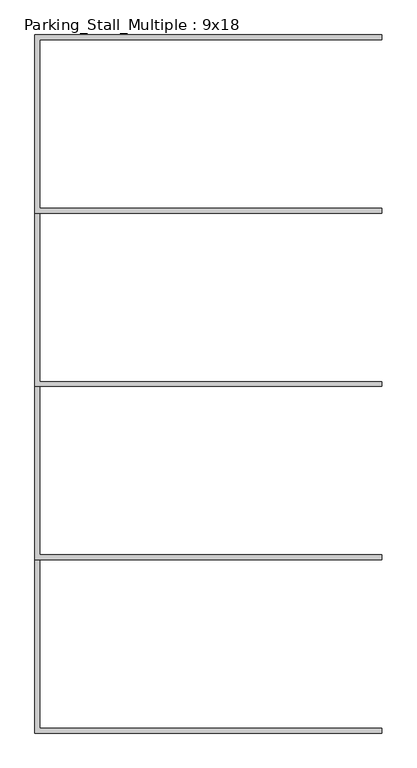
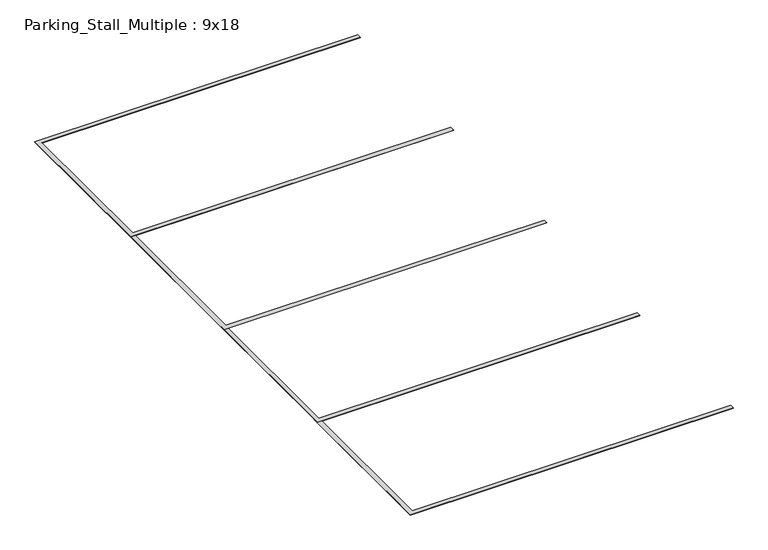
"""IFC4 building model written with IfcOpenShell, lengths in millimetres: proxy geometry, Parking_Stall_Multiple : 9x18."""

from ifc_helpers import new_model, si_unit, origin, origin_with_axes, place, context, project, spatial, polyline, outline, extrude, source, transform, mapped, element, save


def parking_stall_multiple_9x18_ba7214ff(model_context):
    return source(origin(), model_context, "Body", "SweptSolid", [
        extrude(outline(polyline([(5486.4, 8229.6), (0.0, 8229.6), (0.0, 11049.0), (5486.4, 11049.0), (5486.4, 10972.8), (76.2, 10972.8), (76.2, 8305.8), (5486.4, 8305.8), (5486.4, 8229.6)])), origin_with_axes(), (0.0, 0.0, 1.0), 6.35),
        extrude(outline(polyline([(5486.4, 5486.4), (0.0, 5486.4), (0.0, 8305.8), (5486.4, 8305.8), (5486.4, 8229.6), (76.2, 8229.6), (76.2, 5562.6), (5486.4, 5562.6), (5486.4, 5486.4)])), origin_with_axes(), (0.0, 0.0, 1.0), 6.35),
        extrude(outline(polyline([(5486.4, 2743.2), (0.0, 2743.2), (0.0, 5562.6), (5486.4, 5562.6), (5486.4, 5486.4), (76.2, 5486.4), (76.2, 2819.4), (5486.4, 2819.4), (5486.4, 2743.2)])), origin_with_axes(), (0.0, 0.0, 1.0), 6.35),
        extrude(outline(polyline([(5486.4, 0.0), (0.0, 0.0), (0.0, 2819.4), (5486.4, 2819.4), (5486.4, 2743.2), (76.2, 2743.2), (76.2, 76.2), (5486.4, 76.2), (5486.4, 0.0)])), origin_with_axes(), (0.0, 0.0, 1.0), 6.35),
    ])


if __name__ == "__main__":
    model = new_model("IFC4")
    model_context = context("Model", 3, world=origin())
    ifc_project = project(units=[si_unit("LENGTHUNIT", "METRE", prefix="MILLI")], contexts=[model_context])
    site = spatial("IfcSite", under=ifc_project)
    building = spatial("IfcBuilding", under=site)
    placement = place(None, origin())
    parking_stall_multiple_9x18_shape = parking_stall_multiple_9x18_ba7214ff(model_context)
    element("IfcBuildingElementProxy", 1, Name="Parking_Stall_Multiple : 9x18", ObjectType="Parking_Stall_Multiple : 9x18", at=placement, inside=building, context=model_context, shape_type="MappedRepresentation", body=[
        mapped(parking_stall_multiple_9x18_shape, transform((0.0, 0.0, 0.0), x_axis=(1.0, 0.0, 0.0), y_axis=(0.0, 1.0, 0.0), z_axis=(0.0, 0.0, 1.0))),
    ])
    save(model, "model.ifc")

# Revit data of these elements
# Type "Parking_Stall_Multiple : 9x18"
#   Parking_Width_M = 9' - 0"
#   Parking_Run_Length [instance default] = 65' - 0"
#   Parking_Line_Width = 0' - 3"
#   Parking_Length_M = 18' - 0"
#   Single_Parking_Visibility [instance default] = no
#   Parking_ADA_Symbol = no
#   ParkingUnitsArray [instance default] = 7
#   ParkingUnits [instance default] = 7
#   Multiple_Parking_Visibility [instance default] = yes
#   Parking_Line_Material = none
# Element 1 (IfcBuildingElementProxy, "Parking_Stall_Multiple : 9x18")
#   Parking_Run_Length = 36' - 0.74097"
#   ParkingUnitsArray = 4
#   ParkingUnits = 4
